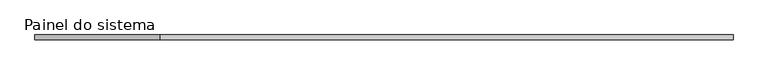
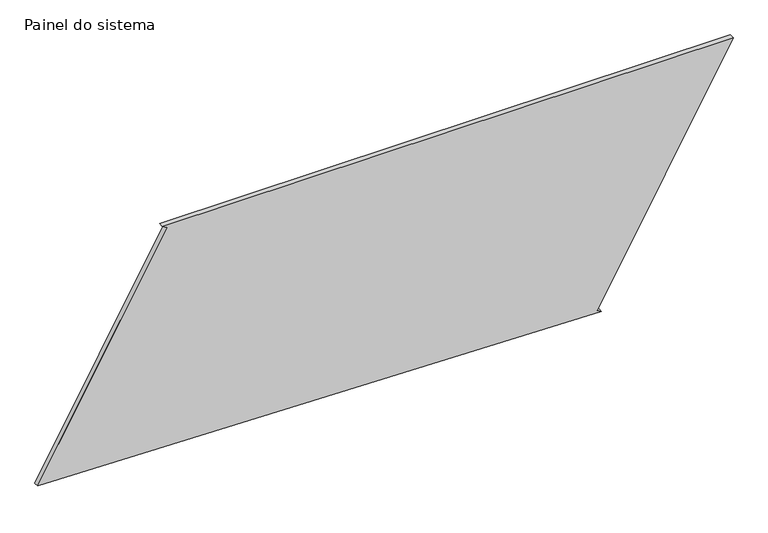
"""IFC4 building model written with IfcOpenShell, lengths in millimetres: plate geometry, Painel do sistema : Envidraçado."""

from ifc_helpers import new_model, si_unit, frame, origin, place, context, project, spatial, polyline, outline, extrude, source, transform, mapped, element, save


def painel_do_sistema_f2a3fa01(model_context):
    return source(origin(), model_context, "Body", "SweptSolid", [
        extrude(outline(polyline([(0.0, 1106.9936182), (12.2820845, 1085.2186234), (1247.2366226, 1781.7889869), (1247.2366226, -1143.1588259), (1234.9545381, -1121.3838311), (64.1175532, -1781.7889869), (0.0, 1106.9936182)])), frame((0.0, 24.5, 0.0), z_axis=(0.0, 1.0, 0.0), x_axis=(0.0, 0.0, 1.0)), (0.0, 0.0, 1.0), 25.0),
    ])


if __name__ == "__main__":
    model = new_model("IFC4")
    model_context = context("Model", 3, world=origin())
    ifc_project = project(units=[si_unit("LENGTHUNIT", "METRE", prefix="MILLI")], contexts=[model_context])
    site = spatial("IfcSite", under=ifc_project)
    building = spatial("IfcBuilding", under=site)
    placement = place(None, origin())
    painel_do_sistema_shape = painel_do_sistema_f2a3fa01(model_context)
    element("IfcPlate", 1, ObjectType="Painel do sistema : Envidraçado", at=placement, inside=building, context=model_context, shape_type="MappedRepresentation", body=[
        mapped(painel_do_sistema_shape, transform((0.0, 0.0, 0.0), x_axis=(1.0, 0.0, 0.0), y_axis=(0.0, 1.0, 0.0), z_axis=(0.0, 0.0, 1.0))),
    ])
    save(model, "model.ifc")

# Revit data of these elements
# Type "Painel do sistema : Envidraçado"
#   Construction Type Id = "GSP4R"
#   Analytic Construction = "Vidraça única Pilkington 1/8 pol"
#   Visual Light Transmittance = 0.9
#   Solar Heat Gain Coefficient = 0.86
#   Heat Transfer Coefficient (U) = 6.7069 W/(m²·K)
# Element 1 (IfcPlate, "Painel do sistema : Envidraçado")
#   Materials on its faces: "Vidro"
# Materials
#   "Vidro": class "Vidro", colour RGB 0 128 192, transparency 0.9, Description = "Vidro de sílica", Cost = 0
